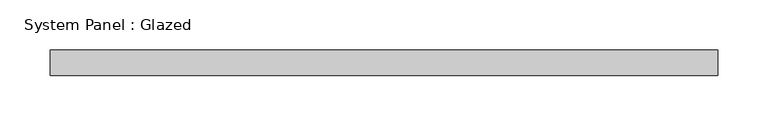
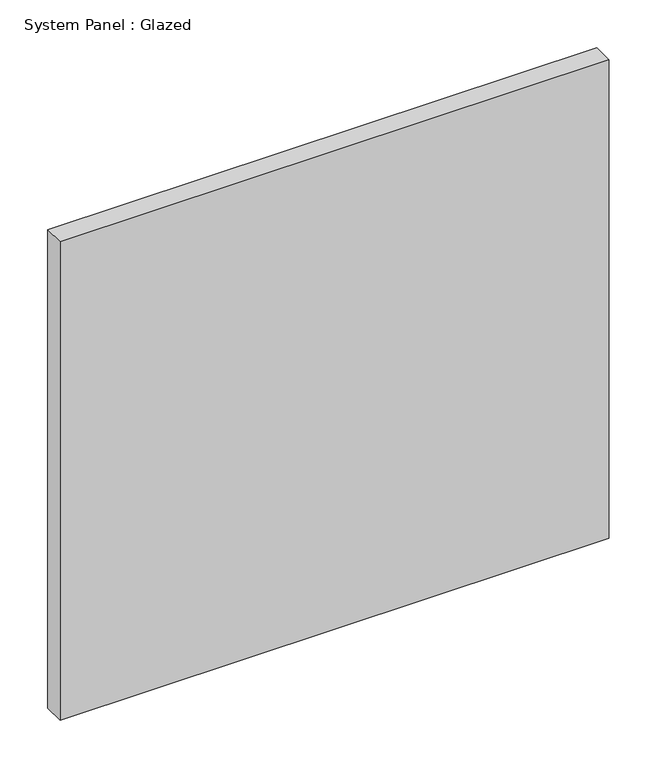
"""IFC4 building model written with IfcOpenShell, lengths in millimetres: plate geometry, System Panel : Glazed."""

from ifc_helpers import new_model, si_unit, origin, origin_with_axes, place, context, project, spatial, polyline, outline, extrude, source, transform, mapped, element, save


def system_panel_glazed_bece7ce1(model_context):
    return source(origin(), model_context, "Body", "SweptSolid", [
        extrude(outline(polyline([(331.132211, 19.05), (-331.132211, 19.05), (-331.132211, 44.45), (331.132211, 44.45), (331.132211, 19.05)])), origin_with_axes(), (0.0, 0.0, 1.0), 609.6),
    ])


if __name__ == "__main__":
    model = new_model("IFC4")
    model_context = context("Model", 3, world=origin())
    ifc_project = project(units=[si_unit("LENGTHUNIT", "METRE", prefix="MILLI")], contexts=[model_context])
    site = spatial("IfcSite", under=ifc_project)
    building = spatial("IfcBuilding", under=site)
    placement = place(None, origin())
    system_panel_glazed_shape = system_panel_glazed_bece7ce1(model_context)
    element("IfcPlate", 1, ObjectType="System Panel : Glazed", at=placement, inside=building, context=model_context, shape_type="MappedRepresentation", body=[
        mapped(system_panel_glazed_shape, transform((0.0, 0.0, 0.0), x_axis=(1.0, 0.0, 0.0), y_axis=(0.0, 1.0, 0.0), z_axis=(0.0, 0.0, 1.0))),
    ])
    save(model, "model.ifc")

# Revit data of these elements
# Element 1 (IfcPlate, "System Panel : Glazed")
#   Materials on its faces: "Glass"
# Materials
#   "Glass": class "Glass", colour RGB 0 128 192, transparency 0.75
